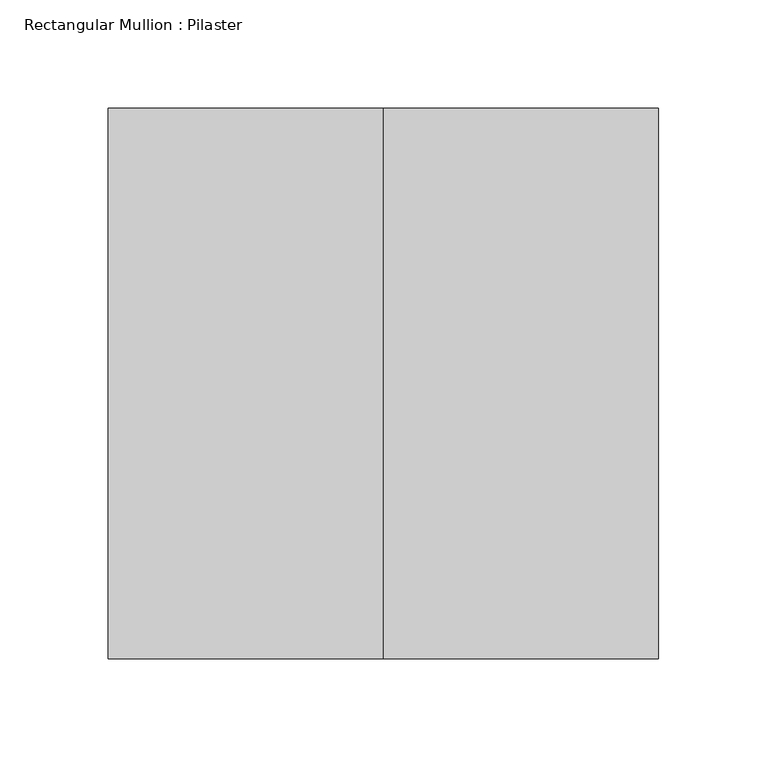
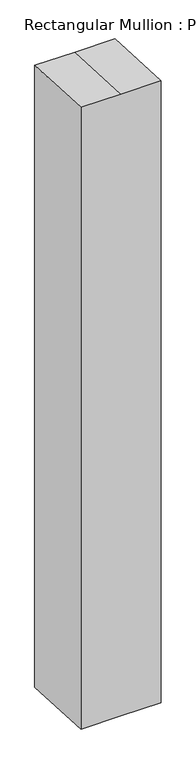
"""IFC4 building model written with IfcOpenShell, lengths in millimetres: member geometry, Rectangular Mullion : Pilaster."""

import ifcopenshell
import ifcopenshell.guid

model = None  # the IFC model being written
_history = None  # IfcOwnerHistory: only IFC2X3 demands one
_inside = {}  # id of a spatial element -> (the spatial element, [elements in it])
_under = {}  # id of a project, library or spatial element -> (it, [spatial elements below it])
_declared = {}  # id of a project -> (the project, [libraries it declares])
_typed = {}  # id of a type object -> (the type object, [elements of that type])
_made_of = {}  # id of a material, layer set ... -> (it, [elements and type objects made of it])


def new_model(schema):
    """Start an empty IFC model of exactly this schema.

    Asked for "IFC4X3", IfcOpenShell would pick the latest addendum, in which some entities
    have other attributes; the version numbers below select the first issue.
    IFC2X3 requires an IfcOwnerHistory on every rooted entity: one is made here for all.
    """
    global model, _history
    if schema == "IFC4X3":
        model = ifcopenshell.file(schema_version=(4, 3, 0, 0))
    else:
        model = ifcopenshell.file(schema=schema)
    _inside.clear()
    _under.clear()
    _declared.clear()
    _typed.clear()
    _made_of.clear()
    _history = None
    if model.schema == "IFC2X3":
        org = make("IfcOrganization", Name="unknown")
        user = make(
            "IfcPersonAndOrganization",
            ThePerson=make("IfcPerson", FamilyName="unknown"),
            TheOrganization=org,
        )
        app = make(
            "IfcApplication",
            ApplicationDeveloper=org,
            Version="unknown",
            ApplicationFullName="unknown",
            ApplicationIdentifier="unknown",
        )
        _history = make(
            "IfcOwnerHistory",
            OwningUser=user,
            OwningApplication=app,
            ChangeAction="ADDED",
            CreationDate=0,
        )
    return model


def make(cls, **values):
    """One entity of the class cls with the attributes given. An attribute that is None is left unset."""
    return model.create_entity(
        cls, **{name: value for name, value in values.items() if value is not None}
    )


def rooted(cls, **values):
    """An entity with a GlobalId (a new one), such as an element, a storey or a relation."""
    return make(cls, GlobalId=ifcopenshell.guid.new(), OwnerHistory=_history, **values)


def si_unit(unit_type, name, prefix=None):
    """IfcSIUnit, for example si_unit("LENGTHUNIT", "METRE", prefix="MILLI")."""
    return make("IfcSIUnit", UnitType=unit_type, Prefix=prefix, Name=name)


def assignment(units):
    """IfcUnitAssignment: the units of a project."""
    return None if units is None else make("IfcUnitAssignment", Units=units)


def point(xyz):
    """IfcCartesianPoint."""
    return None if xyz is None else make("IfcCartesianPoint", Coordinates=xyz)


def direction(xyz):
    """IfcDirection."""
    return None if xyz is None else make("IfcDirection", DirectionRatios=xyz)


def frame(location, z_axis=None, x_axis=None):
    """IfcAxis2Placement3D, a coordinate frame: its origin and axes. An axis left out is left unset."""
    return make(
        "IfcAxis2Placement3D",
        Location=point(location),
        Axis=direction(z_axis),
        RefDirection=direction(x_axis),
    )


def origin():
    """The frame at (0, 0, 0) with its axes left unset."""
    return frame((0.0, 0.0, 0.0))


def place(relative_to, where):
    """IfcLocalPlacement: puts the frame where relative to a parent placement (None: the world)."""
    return make(
        "IfcLocalPlacement", PlacementRelTo=relative_to, RelativePlacement=where
    )


def context(
    kind, dimensions, precision=None, world=None, true_north=None, identifier=None
):
    """IfcGeometricRepresentationContext, for example the 3D "Model" context."""
    return make(
        "IfcGeometricRepresentationContext",
        ContextIdentifier=identifier,
        ContextType=kind,
        CoordinateSpaceDimension=dimensions,
        Precision=precision,
        WorldCoordinateSystem=world,
        TrueNorth=true_north,
    )


def project(units=None, contexts=None):
    """IfcProject with its units and contexts."""
    return rooted(
        "IfcProject",
        Name="project",
        RepresentationContexts=contexts,
        UnitsInContext=assignment(units),
    )


def spatial(cls, under=None, at=None, **own):
    """A site, building, storey or space (cls), placed at a placement, below another one or the project."""
    s = rooted(cls, ObjectPlacement=at, **own)
    if under is not None:
        _under.setdefault(under.id(), (under, []))[1].append(s)
    return s


def faces_of(points, faces, orient=None, outer=None):
    """IfcFace entities. A face is a list of loops; a loop is a list of indices into points, from 0.

    orient and outer hold one flag for each loop. By default every Orientation is true, the
    first loop of a face is its IfcFaceOuterBound and the others are IfcFaceBound.
    """
    made = []
    for i, loops in enumerate(faces):
        bounds = []
        for j, loop in enumerate(loops):
            is_outer = j == 0 if outer is None else outer[i][j]
            bounds.append(
                make(
                    "IfcFaceOuterBound" if is_outer else "IfcFaceBound",
                    Bound=make("IfcPolyLoop", Polygon=[points[k] for k in loop]),
                    Orientation=True if orient is None else orient[i][j],
                )
            )
        made.append(make("IfcFace", Bounds=bounds))
    return made


def faceted_brep(points, faces, orient=None, outer=None, voids=None):
    """IfcFacetedBrep: a solid bounded by flat faces; with voids (closed shells), ...WithVoids."""
    shared = [point(p) for p in points]
    hull = make("IfcClosedShell", CfsFaces=faces_of(shared, faces, orient, outer))
    if voids is None:
        return make("IfcFacetedBrep", Outer=hull)
    return make(
        "IfcFacetedBrepWithVoids",
        Outer=hull,
        Voids=[
            make(cls, CfsFaces=faces_of(shared, fs, o, b)) for cls, fs, o, b in voids
        ],
    )


def shape(context_of_items, identifier, shape_type, items):
    """IfcShapeRepresentation: the items that make up one representation, for example the "Body"."""
    return make(
        "IfcShapeRepresentation",
        ContextOfItems=context_of_items,
        RepresentationIdentifier=identifier,
        RepresentationType=shape_type,
        Items=items,
    )


def source(mapping_origin, context_of_items, identifier, shape_type, items):
    """IfcRepresentationMap: a shape defined once, which mapped items show again and again."""
    return make(
        "IfcRepresentationMap",
        MappingOrigin=mapping_origin,
        MappedRepresentation=shape(context_of_items, identifier, shape_type, items),
    )


def transform(
    local_origin,
    x_axis=None,
    y_axis=None,
    z_axis=None,
    scale=None,
    scale2=None,
    scale3=None,
    uniform=True,
):
    """IfcCartesianTransformationOperator3D, or its non-uniform kind. x_axis, y_axis, z_axis: its Axis1, 2, 3."""
    if uniform:
        return make(
            "IfcCartesianTransformationOperator3D",
            Axis1=direction(x_axis),
            Axis2=direction(y_axis),
            LocalOrigin=point(local_origin),
            Scale=scale,
            Axis3=direction(z_axis),
        )
    return make(
        "IfcCartesianTransformationOperator3DnonUniform",
        Axis1=direction(x_axis),
        Axis2=direction(y_axis),
        LocalOrigin=point(local_origin),
        Scale=scale,
        Axis3=direction(z_axis),
        Scale2=scale2,
        Scale3=scale3,
    )


def mapped(mapping_source, mapping_target):
    """IfcMappedItem: shows the shape of a source again, moved by a transform."""
    return make(
        "IfcMappedItem", MappingSource=mapping_source, MappingTarget=mapping_target
    )


def made_of(thing, what):
    """Note that an element or type object is made of a material, layer set ...; save() writes the relation."""
    if what is not None:
        _made_of.setdefault(what.id(), (what, []))[1].append(thing)
    return thing


def element(
    cls,
    number,
    at=None,
    inside=None,
    cuts=None,
    type_object=None,
    material=None,
    context=None,
    identifier="Body",
    shape_type=None,
    held_by="IfcProductDefinitionShape",
    body=None,
    shapes=None,
    **own,
):
    """One element of the class cls, such as IfcWall. Its Tag is "e" and its number.

    at: its placement. inside: the storey or other place that contains it. cuts: it is an
    opening in that element (IfcRelVoidsElement). A single representation is given by context,
    identifier, shape_type and body (its items); several are given by shapes. held_by: the class
    of the entity that holds the representations. save() writes the other relations.
    """
    e = rooted(cls, Tag="e%d" % number, ObjectPlacement=at, **own)
    if body is not None:
        shapes = [shape(context, identifier, shape_type, body)]
    if shapes is not None:
        e.Representation = make(held_by, Representations=shapes)
    if inside is not None:
        _inside.setdefault(inside.id(), (inside, []))[1].append(e)
    if cuts is not None:
        rooted(
            "IfcRelVoidsElement", RelatingBuildingElement=cuts, RelatedOpeningElement=e
        )
    if type_object is not None:
        _typed.setdefault(type_object.id(), (type_object, []))[1].append(e)
    return made_of(e, material)


def aggregate(whole, parts):
    """IfcRelAggregates: a whole, such as a stair, and the parts it consists of."""
    return rooted("IfcRelAggregates", RelatingObject=whole, RelatedObjects=parts)


def save(model, path):
    """Write the relations noted so far, then the file.

    IfcRelAggregates (storeys below a building ...), IfcRelContainedInSpatialStructure (elements
    in a storey), IfcRelDefinesByType, IfcRelAssociatesMaterial and IfcRelDeclares: one each for
    every whole, place, type object, material and project.
    """
    for whole, parts in _under.values():
        aggregate(whole, parts)
    for where, things in _inside.values():
        rooted(
            "IfcRelContainedInSpatialStructure",
            RelatedElements=things,
            RelatingStructure=where,
        )
    for kind, things in _typed.values():
        rooted("IfcRelDefinesByType", RelatedObjects=things, RelatingType=kind)
    for what, things in _made_of.values():
        rooted("IfcRelAssociatesMaterial", RelatedObjects=things, RelatingMaterial=what)
    for by, libraries in _declared.values():
        rooted("IfcRelDeclares", RelatingContext=by, RelatedDefinitions=libraries)
    model.write(path)


def rectangular_mullion_pilaster_3233f82e(model_context):
    return source(origin(), model_context, "Body", "Brep", [
        faceted_brep([(-127.0, 127.0, -7.074079), (0.0, 127.0, -7.074079), (127.0, 127.0, -7.074079), (127.0, 127.0, -2088.7654929), (0.0, 127.0, -2088.7654929), (-127.0, 127.0, -2088.7654929), (-127.0, -127.0, 6.2374969), (-127.0, -127.0, -2075.4539169), (127.0, -127.0, 6.2374969), (0.0, -127.0, 6.2374969), (0.0, -127.0, -2075.4539169), (127.0, -127.0, -2075.4539169)], [[[0, 1, 2, 3, 4, 5]], [[6, 0, 5, 7]], [[8, 9, 6, 7, 10, 11]], [[2, 8, 11, 3]], [[2, 1, 9, 8]], [[1, 0, 6, 9]], [[3, 11, 10, 4]], [[10, 7, 5, 4]]]),
    ])


if __name__ == "__main__":
    model = new_model("IFC4")
    model_context = context("Model", 3, world=origin())
    ifc_project = project(units=[si_unit("LENGTHUNIT", "METRE", prefix="MILLI")], contexts=[model_context])
    site = spatial("IfcSite", under=ifc_project)
    building = spatial("IfcBuilding", under=site)
    placement = place(None, origin())
    rectangular_mullion_pilaster_shape = rectangular_mullion_pilaster_3233f82e(model_context)
    element("IfcMember", 1, ObjectType="Rectangular Mullion : Pilaster", at=placement, inside=building, context=model_context, shape_type="MappedRepresentation", body=[
        mapped(rectangular_mullion_pilaster_shape, transform((0.0, 0.0, 0.0), x_axis=(1.0, 0.0, 0.0), y_axis=(0.0, 1.0, 0.0), z_axis=(0.0, 0.0, 1.0))),
    ])
    save(model, "model.ifc")

# Revit data of these elements
# Type "Rectangular Mullion : Pilaster"
#   built-in parameter 1007304 = 0.833333 (stored number, unit not read)
#   built-in parameter 1007301 = 0.416667 (stored number, unit not read)
#   built-in parameter 1007300 = 0.416667 (stored number, unit not read)
# Element 1 (IfcMember, "Rectangular Mullion : Pilaster")
#   Materials on its faces: "Aluminum"
# Materials
#   "Aluminum": class "Metal", colour RGB 247 247 247, transparency 0, Description = "Aluminum 6061", Cost = 0
